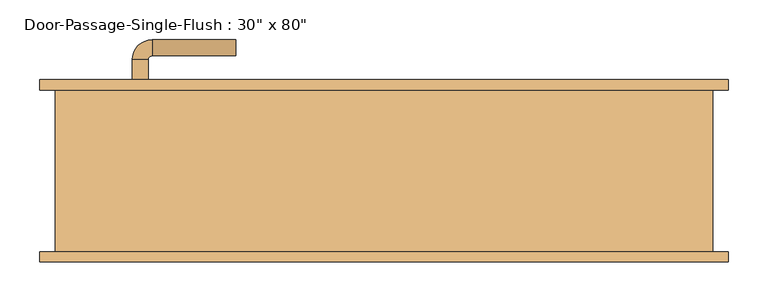
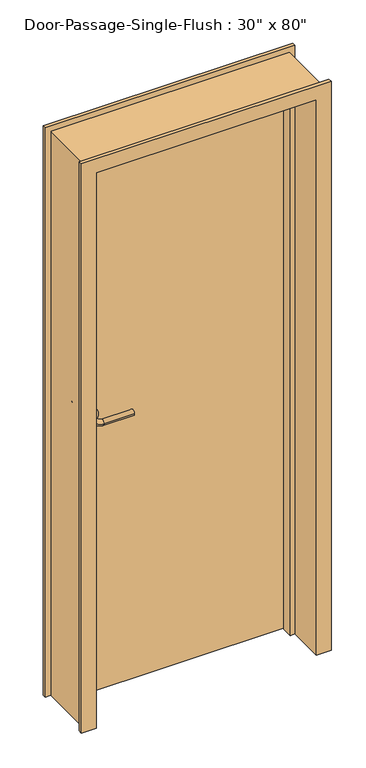
"""IFC4 building model written with IfcOpenShell, lengths in millimetres: door geometry."""

import ifcopenshell
import ifcopenshell.guid

model = None  # the IFC model being written
_history = None  # IfcOwnerHistory: only IFC2X3 demands one
_inside = {}  # id of a spatial element -> (the spatial element, [elements in it])
_under = {}  # id of a project, library or spatial element -> (it, [spatial elements below it])
_declared = {}  # id of a project -> (the project, [libraries it declares])
_typed = {}  # id of a type object -> (the type object, [elements of that type])
_made_of = {}  # id of a material, layer set ... -> (it, [elements and type objects made of it])


def new_model(schema):
    """Start an empty IFC model of exactly this schema.

    Asked for "IFC4X3", IfcOpenShell would pick the latest addendum, in which some entities
    have other attributes; the version numbers below select the first issue.
    IFC2X3 requires an IfcOwnerHistory on every rooted entity: one is made here for all.
    """
    global model, _history
    if schema == "IFC4X3":
        model = ifcopenshell.file(schema_version=(4, 3, 0, 0))
    else:
        model = ifcopenshell.file(schema=schema)
    _inside.clear()
    _under.clear()
    _declared.clear()
    _typed.clear()
    _made_of.clear()
    _history = None
    if model.schema == "IFC2X3":
        org = make("IfcOrganization", Name="unknown")
        user = make(
            "IfcPersonAndOrganization",
            ThePerson=make("IfcPerson", FamilyName="unknown"),
            TheOrganization=org,
        )
        app = make(
            "IfcApplication",
            ApplicationDeveloper=org,
            Version="unknown",
            ApplicationFullName="unknown",
            ApplicationIdentifier="unknown",
        )
        _history = make(
            "IfcOwnerHistory",
            OwningUser=user,
            OwningApplication=app,
            ChangeAction="ADDED",
            CreationDate=0,
        )
    return model


def make(cls, **values):
    """One entity of the class cls with the attributes given. An attribute that is None is left unset."""
    return model.create_entity(
        cls, **{name: value for name, value in values.items() if value is not None}
    )


def rooted(cls, **values):
    """An entity with a GlobalId (a new one), such as an element, a storey or a relation."""
    return make(cls, GlobalId=ifcopenshell.guid.new(), OwnerHistory=_history, **values)


def si_unit(unit_type, name, prefix=None):
    """IfcSIUnit, for example si_unit("LENGTHUNIT", "METRE", prefix="MILLI")."""
    return make("IfcSIUnit", UnitType=unit_type, Prefix=prefix, Name=name)


def assignment(units):
    """IfcUnitAssignment: the units of a project."""
    return None if units is None else make("IfcUnitAssignment", Units=units)


def point(xyz):
    """IfcCartesianPoint."""
    return None if xyz is None else make("IfcCartesianPoint", Coordinates=xyz)


def direction(xyz):
    """IfcDirection."""
    return None if xyz is None else make("IfcDirection", DirectionRatios=xyz)


def frame(location, z_axis=None, x_axis=None):
    """IfcAxis2Placement3D, a coordinate frame: its origin and axes. An axis left out is left unset."""
    return make(
        "IfcAxis2Placement3D",
        Location=point(location),
        Axis=direction(z_axis),
        RefDirection=direction(x_axis),
    )


def frame_2d(location, x_axis=None):
    """IfcAxis2Placement2D, a coordinate frame in the plane: its origin and x axis."""
    return make(
        "IfcAxis2Placement2D", Location=point(location), RefDirection=direction(x_axis)
    )


def origin():
    """The frame at (0, 0, 0) with its axes left unset."""
    return frame((0.0, 0.0, 0.0))


def origin_with_axes():
    """The frame at (0, 0, 0) with the z axis (0, 0, 1) and the x axis (1, 0, 0) written out."""
    return frame((0.0, 0.0, 0.0), z_axis=(0.0, 0.0, 1.0), x_axis=(1.0, 0.0, 0.0))


def place(relative_to, where):
    """IfcLocalPlacement: puts the frame where relative to a parent placement (None: the world)."""
    return make(
        "IfcLocalPlacement", PlacementRelTo=relative_to, RelativePlacement=where
    )


def context(
    kind, dimensions, precision=None, world=None, true_north=None, identifier=None
):
    """IfcGeometricRepresentationContext, for example the 3D "Model" context."""
    return make(
        "IfcGeometricRepresentationContext",
        ContextIdentifier=identifier,
        ContextType=kind,
        CoordinateSpaceDimension=dimensions,
        Precision=precision,
        WorldCoordinateSystem=world,
        TrueNorth=true_north,
    )


def project(units=None, contexts=None):
    """IfcProject with its units and contexts."""
    return rooted(
        "IfcProject",
        Name="project",
        RepresentationContexts=contexts,
        UnitsInContext=assignment(units),
    )


def spatial(cls, under=None, at=None, **own):
    """A site, building, storey or space (cls), placed at a placement, below another one or the project."""
    s = rooted(cls, ObjectPlacement=at, **own)
    if under is not None:
        _under.setdefault(under.id(), (under, []))[1].append(s)
    return s


def polyline(points):
    """IfcPolyline through the points."""
    return make("IfcPolyline", Points=[point(p) for p in points])


def circle_curve(where, radius):
    """IfcCircle in the frame where."""
    return make("IfcCircle", Position=where, Radius=radius)


def ellipse_curve(where, semi_axis1, semi_axis2):
    """IfcEllipse in the frame where."""
    return make(
        "IfcEllipse", Position=where, SemiAxis1=semi_axis1, SemiAxis2=semi_axis2
    )


def trimmed(basis, trim1, trim2, sense, master):
    """IfcTrimmedCurve: the piece of a basis curve between two trims."""
    return make(
        "IfcTrimmedCurve",
        BasisCurve=basis,
        Trim1=trim1,
        Trim2=trim2,
        SenseAgreement=sense,
        MasterRepresentation=master,
    )


def segment(curve, same_sense, transition):
    """IfcCompositeCurveSegment."""
    return make(
        "IfcCompositeCurveSegment",
        Transition=transition,
        SameSense=same_sense,
        ParentCurve=curve,
    )


def composite_curve(segments, self_intersect=None):
    """IfcCompositeCurve: segments joined end to end."""
    return make("IfcCompositeCurve", Segments=segments, SelfIntersect=self_intersect)


def outline(outer, holes=None, kind="AREA"):
    """IfcArbitraryClosedProfileDef: a profile drawn as a closed curve; with holes, ...WithVoids."""
    if holes is None:
        return make("IfcArbitraryClosedProfileDef", ProfileType=kind, OuterCurve=outer)
    return make(
        "IfcArbitraryProfileDefWithVoids",
        ProfileType=kind,
        OuterCurve=outer,
        InnerCurves=holes,
    )


def extrude(swept, where, along, depth):
    """IfcExtrudedAreaSolid: the profile swept, set in the frame where, extruded along a direction by depth."""
    return make(
        "IfcExtrudedAreaSolid",
        SweptArea=swept,
        Position=where,
        ExtrudedDirection=direction(along),
        Depth=depth,
    )


def faces_of(points, faces, orient=None, outer=None):
    """IfcFace entities. A face is a list of loops; a loop is a list of indices into points, from 0.

    orient and outer hold one flag for each loop. By default every Orientation is true, the
    first loop of a face is its IfcFaceOuterBound and the others are IfcFaceBound.
    """
    made = []
    for i, loops in enumerate(faces):
        bounds = []
        for j, loop in enumerate(loops):
            is_outer = j == 0 if outer is None else outer[i][j]
            bounds.append(
                make(
                    "IfcFaceOuterBound" if is_outer else "IfcFaceBound",
                    Bound=make("IfcPolyLoop", Polygon=[points[k] for k in loop]),
                    Orientation=True if orient is None else orient[i][j],
                )
            )
        made.append(make("IfcFace", Bounds=bounds))
    return made


def faceted_brep(points, faces, orient=None, outer=None, voids=None):
    """IfcFacetedBrep: a solid bounded by flat faces; with voids (closed shells), ...WithVoids."""
    shared = [point(p) for p in points]
    hull = make("IfcClosedShell", CfsFaces=faces_of(shared, faces, orient, outer))
    if voids is None:
        return make("IfcFacetedBrep", Outer=hull)
    return make(
        "IfcFacetedBrepWithVoids",
        Outer=hull,
        Voids=[
            make(cls, CfsFaces=faces_of(shared, fs, o, b)) for cls, fs, o, b in voids
        ],
    )


def shape(context_of_items, identifier, shape_type, items):
    """IfcShapeRepresentation: the items that make up one representation, for example the "Body"."""
    return make(
        "IfcShapeRepresentation",
        ContextOfItems=context_of_items,
        RepresentationIdentifier=identifier,
        RepresentationType=shape_type,
        Items=items,
    )


def source(mapping_origin, context_of_items, identifier, shape_type, items):
    """IfcRepresentationMap: a shape defined once, which mapped items show again and again."""
    return make(
        "IfcRepresentationMap",
        MappingOrigin=mapping_origin,
        MappedRepresentation=shape(context_of_items, identifier, shape_type, items),
    )


def transform(
    local_origin,
    x_axis=None,
    y_axis=None,
    z_axis=None,
    scale=None,
    scale2=None,
    scale3=None,
    uniform=True,
):
    """IfcCartesianTransformationOperator3D, or its non-uniform kind. x_axis, y_axis, z_axis: its Axis1, 2, 3."""
    if uniform:
        return make(
            "IfcCartesianTransformationOperator3D",
            Axis1=direction(x_axis),
            Axis2=direction(y_axis),
            LocalOrigin=point(local_origin),
            Scale=scale,
            Axis3=direction(z_axis),
        )
    return make(
        "IfcCartesianTransformationOperator3DnonUniform",
        Axis1=direction(x_axis),
        Axis2=direction(y_axis),
        LocalOrigin=point(local_origin),
        Scale=scale,
        Axis3=direction(z_axis),
        Scale2=scale2,
        Scale3=scale3,
    )


def mapped(mapping_source, mapping_target):
    """IfcMappedItem: shows the shape of a source again, moved by a transform."""
    return make(
        "IfcMappedItem", MappingSource=mapping_source, MappingTarget=mapping_target
    )


def made_of(thing, what):
    """Note that an element or type object is made of a material, layer set ...; save() writes the relation."""
    if what is not None:
        _made_of.setdefault(what.id(), (what, []))[1].append(thing)
    return thing


def element(
    cls,
    number,
    at=None,
    inside=None,
    cuts=None,
    type_object=None,
    material=None,
    context=None,
    identifier="Body",
    shape_type=None,
    held_by="IfcProductDefinitionShape",
    body=None,
    shapes=None,
    **own,
):
    """One element of the class cls, such as IfcWall. Its Tag is "e" and its number.

    at: its placement. inside: the storey or other place that contains it. cuts: it is an
    opening in that element (IfcRelVoidsElement). A single representation is given by context,
    identifier, shape_type and body (its items); several are given by shapes. held_by: the class
    of the entity that holds the representations. save() writes the other relations.
    """
    e = rooted(cls, Tag="e%d" % number, ObjectPlacement=at, **own)
    if body is not None:
        shapes = [shape(context, identifier, shape_type, body)]
    if shapes is not None:
        e.Representation = make(held_by, Representations=shapes)
    if inside is not None:
        _inside.setdefault(inside.id(), (inside, []))[1].append(e)
    if cuts is not None:
        rooted(
            "IfcRelVoidsElement", RelatingBuildingElement=cuts, RelatedOpeningElement=e
        )
    if type_object is not None:
        _typed.setdefault(type_object.id(), (type_object, []))[1].append(e)
    return made_of(e, material)


def aggregate(whole, parts):
    """IfcRelAggregates: a whole, such as a stair, and the parts it consists of."""
    return rooted("IfcRelAggregates", RelatingObject=whole, RelatedObjects=parts)


def save(model, path):
    """Write the relations noted so far, then the file.

    IfcRelAggregates (storeys below a building ...), IfcRelContainedInSpatialStructure (elements
    in a storey), IfcRelDefinesByType, IfcRelAssociatesMaterial and IfcRelDeclares: one each for
    every whole, place, type object, material and project.
    """
    for whole, parts in _under.values():
        aggregate(whole, parts)
    for where, things in _inside.values():
        rooted(
            "IfcRelContainedInSpatialStructure",
            RelatedElements=things,
            RelatingStructure=where,
        )
    for kind, things in _typed.values():
        rooted("IfcRelDefinesByType", RelatedObjects=things, RelatingType=kind)
    for what, things in _made_of.values():
        rooted("IfcRelAssociatesMaterial", RelatedObjects=things, RelatingMaterial=what)
    for by, libraries in _declared.values():
        rooted("IfcRelDeclares", RelatingContext=by, RelatedDefinitions=libraries)
    model.write(path)


def plane_surface(at):
    """IfcPlane: the flat surface through the origin of the frame at, square to its z axis."""
    return make("IfcPlane", Position=at)


def cylinder_surface(at, radius):
    """IfcCylindricalSurface: all points at the distance radius from the z axis of the frame at."""
    return make("IfcCylindricalSurface", Position=at, Radius=radius)


def revolved_surface(curve, axis_point, axis_direction):
    """IfcSurfaceOfRevolution: the curve turned about the line through axis_point along axis_direction."""
    return make(
        "IfcSurfaceOfRevolution",
        SweptCurve=make("IfcArbitraryOpenProfileDef", ProfileType="CURVE", Curve=curve),
        AxisPosition=make("IfcAxis1Placement", Location=point(axis_point), Axis=direction(axis_direction)),
    )


def advanced_brep(points, edges, surfaces, faces):
    """IfcAdvancedBrep: a solid bounded by faces that lie on surfaces and meet in shared edges.

    An edge is (start, end): straight between two places in points (the first is 0);
    or (start, end, curve); or (start, end, curve, False) where it runs against its curve.
    A face is (place in surfaces, loops), or (place, loops, False) where it looks against
    its surface's normal. A loop lists edges by number (the first is 1), with a minus sign
    where the edge is run from its end to its start. The first loop is the outer one.
    """
    corners = [point(p) for p in points]
    vertices = [make("IfcVertexPoint", VertexGeometry=c) for c in corners]
    made = []
    for start, end, *more in edges:
        made.append(
            make(
                "IfcEdgeCurve",
                EdgeStart=vertices[start],
                EdgeEnd=vertices[end],
                EdgeGeometry=more[0] if more else make("IfcPolyline", Points=[corners[start], corners[end]]),
                SameSense=more[1] if len(more) > 1 else True,
            )
        )
    hull = []
    for where, loops, *sense in faces:
        bounds = []
        for j, loop in enumerate(loops):
            ring = [make("IfcOrientedEdge", EdgeElement=made[abs(k) - 1], Orientation=k > 0) for k in loop]
            bounds.append(
                make(
                    "IfcFaceOuterBound" if j == 0 else "IfcFaceBound",
                    Bound=make("IfcEdgeLoop", EdgeList=ring),
                    Orientation=True,
                )
            )
        hull.append(make("IfcAdvancedFace", Bounds=bounds, FaceSurface=surfaces[where], SameSense=sense[0] if sense else True))
    return make("IfcAdvancedBrep", Outer=make("IfcClosedShell", CfsFaces=hull))


def door_053fcaeb(model_context):
    return source(origin(), model_context, "Body", "SolidModel", [
        advanced_brep(
        [(-315.990625, 55.5, 1016.0), (-295.990625, 55.5, 1016.0), (-295.990625, 25.5, 1016.0), (-315.990625, 25.5, 1016.0), (-290.990625, 20.5, 1016.0), (-290.990625, 0.5, 1016.0), (-185.990625, 0.5, 1016.0), (-185.990625, 20.5, 1016.0)],
        [
            (0, 1, circle_curve(frame((-305.990625, 55.5, 1016.0), z_axis=(0.0, 1.0, 0.0), x_axis=(1.0, 0.0, 0.0)), 10.0)),
            (1, 0, circle_curve(frame((-305.990625, 55.5, 1016.0), z_axis=(0.0, 1.0, 0.0), x_axis=(1.0, 0.0, 0.0)), 10.0)),
            (1, 2),
            (2, 3, circle_curve(frame((-305.990625, 25.5, 1016.0), z_axis=(0.0, 1.0, 0.0), x_axis=(1.0, 0.0, 0.0)), 10.0)),
            (3, 0),
            (3, 2, circle_curve(frame((-305.990625, 25.5, 1016.0), z_axis=(0.0, 1.0, 0.0), x_axis=(1.0, 0.0, 0.0)), 10.0)),
            (4, 5, circle_curve(frame((-290.990625, 10.5, 1016.0), z_axis=(-1.0, 0.0, 0.0), x_axis=(0.0, 1.0, 0.0)), 10.0)),
            (5, 3, circle_curve(frame((-290.990625, 25.5, 1016.0), z_axis=(0.0, 0.0, -1.0), x_axis=(-1.0, 0.0, 0.0)), 25.0)),
            (2, 4, circle_curve(frame((-290.990625, 25.5, 1016.0), z_axis=(0.0, 0.0, 1.0), x_axis=(-1.0, 0.0, 0.0)), 5.0)),
            (5, 4, circle_curve(frame((-290.990625, 10.5, 1016.0), z_axis=(-1.0, 0.0, 0.0), x_axis=(0.0, 1.0, 0.0)), 10.0)),
            (6, 7, circle_curve(frame((-185.990625, 10.5, 1016.0), z_axis=(1.0, 0.0, 0.0), x_axis=(0.0, 1.0, 0.0)), 10.0)),
            (7, 6, circle_curve(frame((-185.990625, 10.5, 1016.0), z_axis=(1.0, 0.0, 0.0), x_axis=(0.0, 1.0, 0.0)), 10.0)),
            (4, 7),
            (6, 5),
        ],
        [
            plane_surface(frame((-305.990625, 55.5, 1016.0), z_axis=(0.0, 1.0, 0.0), x_axis=(0.0, 0.0, 1.0))),
            cylinder_surface(frame((-305.990625, 55.5, 1016.0), z_axis=(0.0, 1.0, 0.0), x_axis=(1.0, 0.0, 0.0)), 10.0),
            revolved_surface(trimmed(ellipse_curve(frame((-305.990625, 25.5, 1016.0), z_axis=(0.0, -1.0, 0.0), x_axis=(1.0, 0.0, 0.0)), 10.0, 10.0), [point((-315.990625, 25.5, 1016.0))], [point((-295.990625, 25.5, 1016.0))], True, "CARTESIAN"), (-290.990625, 25.5, 1016.0), (0.0, 0.0, -1.0)),
            revolved_surface(trimmed(ellipse_curve(frame((-305.990625, 25.5, 1016.0), z_axis=(0.0, -1.0, 0.0), x_axis=(1.0, 0.0, 0.0)), 10.0, 10.0), [point((-295.990625, 25.5, 1016.0))], [point((-315.990625, 25.5, 1016.0))], True, "CARTESIAN"), (-290.990625, 25.5, 1016.0), (0.0, 0.0, -1.0)),
            plane_surface(frame((-185.990625, 10.5, 1016.0), z_axis=(1.0, 0.0, 0.0), x_axis=(0.0, 0.0, 1.0))),
            cylinder_surface(frame((-290.990625, 10.5, 1016.0), z_axis=(-1.0, 0.0, 0.0), x_axis=(0.0, 1.0, 0.0)), 10.0),
        ],
        [
            (0, [[1, 2]]),
            (1, [[3, 4, 5, -2]]),
            (1, [[-5, 6, -3, -1]]),
            (2, [[7, 8, -4, 9]]),
            (3, [[10, -9, -6, -8]]),
            (4, [[11, 12]]),
            (5, [[13, -11, 14, -7]]),
            (5, [[-14, -12, -13, -10]]),
        ],
    ),
        extrude(outline(composite_curve([segment(trimmed(circle_curve(frame_2d((1016.0, -308.490625)), 30.0), [point((1016.0, -338.490625))], [point((1016.0, -278.490625))], False, "CARTESIAN"), True, "CONTINUOUS"), segment(trimmed(circle_curve(frame_2d((1016.0, -308.490625)), 30.0), [point((1016.0, -278.490625))], [point((1016.0, -338.490625))], False, "CARTESIAN"), True, "CONTINUOUS")], self_intersect=False)), frame((0.0, 55.5, 0.0), z_axis=(0.0, 1.0, 0.0), x_axis=(0.0, 0.0, 1.0)), (0.0, 0.0, 1.0), 8.0),
        advanced_brep(
        [(-315.990625, 115.95, 1016.0), (-295.990625, 115.95, 1016.0), (-315.990625, 145.95, 1016.0), (-295.990625, 145.95, 1016.0), (-290.990625, 150.95, 1016.0), (-290.990625, 170.95, 1016.0), (-185.990625, 170.95, 1016.0), (-185.990625, 150.95, 1016.0)],
        [
            (0, 1, circle_curve(frame((-305.990625, 115.95, 1016.0), z_axis=(0.0, -1.0, 0.0), x_axis=(1.0, 0.0, 0.0)), 10.0)),
            (1, 0, circle_curve(frame((-305.990625, 115.95, 1016.0), z_axis=(0.0, -1.0, 0.0), x_axis=(1.0, 0.0, 0.0)), 10.0)),
            (0, 2),
            (2, 3, circle_curve(frame((-305.990625, 145.95, 1016.0), z_axis=(0.0, -1.0, 0.0), x_axis=(1.0, 0.0, 0.0)), 10.0)),
            (3, 1),
            (3, 2, circle_curve(frame((-305.990625, 145.95, 1016.0), z_axis=(0.0, -1.0, 0.0), x_axis=(1.0, 0.0, 0.0)), 10.0)),
            (4, 3, circle_curve(frame((-290.990625, 145.95, 1016.0), z_axis=(0.0, 0.0, 1.0), x_axis=(-1.0, 0.0, 0.0)), 5.0)),
            (2, 5, circle_curve(frame((-290.990625, 145.95, 1016.0), z_axis=(0.0, 0.0, -1.0), x_axis=(-1.0, 0.0, 0.0)), 25.0)),
            (5, 4, circle_curve(frame((-290.990625, 160.95, 1016.0), z_axis=(-1.0, 0.0, 0.0), x_axis=(0.0, -1.0, 0.0)), 10.0)),
            (4, 5, circle_curve(frame((-290.990625, 160.95, 1016.0), z_axis=(-1.0, 0.0, 0.0), x_axis=(0.0, -1.0, 0.0)), 10.0)),
            (6, 7, circle_curve(frame((-185.990625, 160.95, 1016.0), z_axis=(1.0, 0.0, 0.0), x_axis=(0.0, -1.0, 0.0)), 10.0)),
            (7, 6, circle_curve(frame((-185.990625, 160.95, 1016.0), z_axis=(1.0, 0.0, 0.0), x_axis=(0.0, -1.0, 0.0)), 10.0)),
            (5, 6),
            (7, 4),
        ],
        [
            plane_surface(frame((-305.990625, 115.95, 1016.0), z_axis=(0.0, -1.0, 0.0), x_axis=(0.0, 0.0, 1.0))),
            cylinder_surface(frame((-305.990625, 115.95, 1016.0), z_axis=(0.0, -1.0, 0.0), x_axis=(1.0, 0.0, 0.0)), 10.0),
            revolved_surface(trimmed(ellipse_curve(frame((-305.990625, 145.95, 1016.0), z_axis=(0.0, -1.0, 0.0), x_axis=(1.0, 0.0, 0.0)), 10.0, 10.0), [point((-315.990625, 145.95, 1016.0))], [point((-295.990625, 145.95, 1016.0))], True, "CARTESIAN"), (-290.990625, 145.95, 1016.0), (0.0, 0.0, -1.0)),
            revolved_surface(trimmed(ellipse_curve(frame((-305.990625, 145.95, 1016.0), z_axis=(0.0, -1.0, 0.0), x_axis=(1.0, 0.0, 0.0)), 10.0, 10.0), [point((-295.990625, 145.95, 1016.0))], [point((-315.990625, 145.95, 1016.0))], True, "CARTESIAN"), (-290.990625, 145.95, 1016.0), (0.0, 0.0, -1.0)),
            plane_surface(frame((-185.990625, 160.95, 1016.0), z_axis=(1.0, 0.0, 0.0), x_axis=(0.0, 0.0, 1.0))),
            cylinder_surface(frame((-290.990625, 160.95, 1016.0), z_axis=(-1.0, 0.0, 0.0), x_axis=(0.0, -1.0, 0.0)), 10.0),
        ],
        [
            (0, [[1, 2]]),
            (1, [[-1, 3, 4, 5]]),
            (1, [[-2, -5, 6, -3]]),
            (2, [[7, -4, 8, 9]]),
            (3, [[-8, -6, -7, 10]]),
            (4, [[11, 12]]),
            (5, [[-9, 13, -12, 14]]),
            (5, [[-10, -14, -11, -13]]),
        ],
    ),
        extrude(outline(composite_curve([segment(trimmed(circle_curve(frame_2d((1016.0, -308.490625)), 30.0), [point((1016.0, -338.490625))], [point((1016.0, -278.490625))], False, "CARTESIAN"), True, "CONTINUOUS"), segment(trimmed(circle_curve(frame_2d((1016.0, -308.490625)), 30.0), [point((1016.0, -278.490625))], [point((1016.0, -338.490625))], False, "CARTESIAN"), True, "CONTINUOUS")], self_intersect=False)), frame((0.0, 107.95, 0.0), z_axis=(0.0, 1.0, 0.0), x_axis=(0.0, 0.0, 1.0)), (0.0, 0.0, 1.0), 8.0),
        faceted_brep([(381.0, 120.65, 0.0), (431.8, 120.65, 0.0), (431.8, 107.95, 0.0), (412.75, 107.95, 0.0), (412.75, -95.25, 0.0), (431.8, -95.25, 0.0), (431.8, -107.95, 0.0), (381.0, -107.95, 0.0), (381.0, 20.6375, 0.0), (365.125, 20.6375, 0.0), (365.125, 58.7375, 0.0), (381.0, 58.7375, 0.0), (381.0, 120.65, 2032.0), (-381.0, 120.65, 2032.0), (-381.0, 120.65, 0.0), (-431.8, 120.65, 0.0), (-431.8, 120.65, 2082.8), (431.8, 120.65, 2082.8), (431.8, 107.95, 2082.8), (-431.8, 107.95, 2082.8), (-431.8, 107.95, 0.0), (-412.75, 107.95, 0.0), (-412.75, 107.95, 2063.75), (412.75, 107.95, 2063.75), (412.75, -95.25, 2063.75), (-412.75, -95.25, 2063.75), (-412.75, -95.25, 0.0), (-431.8, -95.25, 0.0), (-431.8, -95.25, 2082.8), (431.8, -95.25, 2082.8), (431.8, -107.95, 2082.8), (-431.8, -107.95, 2082.8), (-431.8, -107.95, 0.0), (-381.0, -107.95, 0.0), (-381.0, -107.95, 2032.0), (381.0, -107.95, 2032.0), (381.0, 20.6375, 2032.0), (-381.0, 20.6375, 2032.0), (-381.0, 20.6375, 0.0), (-365.125, 20.6375, 0.0), (-365.125, 20.6375, 2016.125), (365.125, 20.6375, 2016.125), (365.125, 58.7375, 2016.125), (-365.125, 58.7375, 2016.125), (-365.125, 58.7375, 0.0), (-381.0, 58.7375, 0.0), (-381.0, 58.7375, 2032.0), (381.0, 58.7375, 2032.0)], [[[0, 1, 2, 3, 4, 5, 6, 7, 8, 9, 10, 11]], [[1, 0, 12, 13, 14, 15, 16, 17]], [[2, 1, 17, 18]], [[3, 2, 18, 19, 20, 21, 22, 23]], [[4, 3, 23, 24]], [[5, 4, 24, 25, 26, 27, 28, 29]], [[6, 5, 29, 30]], [[7, 6, 30, 31, 32, 33, 34, 35]], [[8, 7, 35, 36]], [[9, 8, 36, 37, 38, 39, 40, 41]], [[10, 9, 41, 42]], [[11, 10, 42, 43, 44, 45, 46, 47]], [[0, 11, 47, 12]], [[18, 17, 16, 19]], [[24, 23, 22, 25]], [[30, 29, 28, 31]], [[36, 35, 34, 37]], [[42, 41, 40, 43]], [[12, 47, 46, 13]], [[14, 45, 44, 39, 38, 33, 32, 27, 26, 21, 20, 15]], [[19, 16, 15, 20]], [[25, 22, 21, 26]], [[31, 28, 27, 32]], [[37, 34, 33, 38]], [[43, 40, 39, 44]], [[13, 46, 45, 14]]]),
        extrude(outline(polyline([(381.0, 63.5), (-381.0, 63.5), (-381.0, 107.95), (381.0, 107.95), (381.0, 63.5)])), origin_with_axes(), (0.0, 0.0, 1.0), 2032.0),
    ])


if __name__ == "__main__":
    model = new_model("IFC4")
    model_context = context("Model", 3, world=origin())
    ifc_project = project(units=[si_unit("LENGTHUNIT", "METRE", prefix="MILLI")], contexts=[model_context])
    site = spatial("IfcSite", under=ifc_project)
    building = spatial("IfcBuilding", under=site)
    placement = place(None, origin())
    door_shape = door_053fcaeb(model_context)
    element("IfcDoor", 1, ObjectType="Door-Passage-Single-Flush : 30\" x 80\"", at=placement, inside=building, context=model_context, shape_type="MappedRepresentation", body=[
        mapped(door_shape, transform((0.0, 0.0, 0.0), x_axis=(1.0, 0.0, 0.0), y_axis=(0.0, 1.0, 0.0), z_axis=(0.0, 0.0, 1.0))),
    ])
    save(model, "model.ifc")

# Revit data of these elements
# Project information
#   Project Issue Date = "Issue Date"
#   Project Status = "Project Status"
#   Client Name = "Owner"
#   Project Address = "Enter address here"
#   Project Name = "Project Name"
#   Project Number = "Project Number"
# Type "Door-Passage-Single-Flush : 30\" x 80\""
#   Type Mark = "16"
#   Assembly Code = "B2030200"
#   Analytic Construction = "Wooden"
#   Thickness = 0' - 1 3/4"
#   Thermal Resistance (R) = 2.5876 (h·ft²·°F)/BTU
#   Swing Angle [instance default] = 90.00°
#   Strike Height = 3' - 4"
#   Rough Width [instance default] = 2' - 10"
#   Rough Height [instance default] = 7' - 0"
#   MF Opening Height [instance default] = 0' - 4"
#   MF Opening Width [instance default] = 0' - 4"
#   Inset Calculate [instance default] = 0' - 4"
#   Masonry Inset [instance default] = 0' - 1"
#   Height = 6' - 8"
#   Width = 2' - 6"
#   Heat Transfer Coefficient (U) = 0.3865 BTU/(h·ft²·°F)
#   Masonry Frame Depth = 0' - 5 3/4"
#   Masonry Frame [instance default] = yes
#   Function = 1
#   Dry Wall Frame [instance default] = no
#   Panel Material = Wood - Birch
#   Frame Material = Metal - Paint Finish - Grey
#   Door Handle Material = Aluminum
#   Visual Light Transmittance = 0
#   Solar Heat Gain Coefficient = 0
#   Wall Closure = (empty or 0)
# Element 1 (IfcDoor, "Door-Passage-Single-Flush : 30\" x 80\"")
#   Rough Width = 2' - 8 1/2"
#   Rough Height = 6' - 9 1/4"
#   MF Opening Height = 0' - 1 1/4"
#   MF Opening Width = 0' - 2 1/2"
#   Inset Calculate = 0' - 3"
#   Masonry Frame = no
#   Dry Wall Frame = yes
#   Materials on its faces: "Metal - Paint Finish - Grey", "Aluminum", "Wood - Birch"
# Materials
#   "Wood - Birch": class "Wood", colour RGB 166 116 52, transparency 0, Cost = 0
#   "Metal - Paint Finish - Grey": class "Paint", colour RGB 104 104 104, transparency 0, Cost = 0
#   "Aluminum": class "Metal", colour RGB 247 247 247, transparency 0, Description = "Aluminum 6061", Cost = 0
